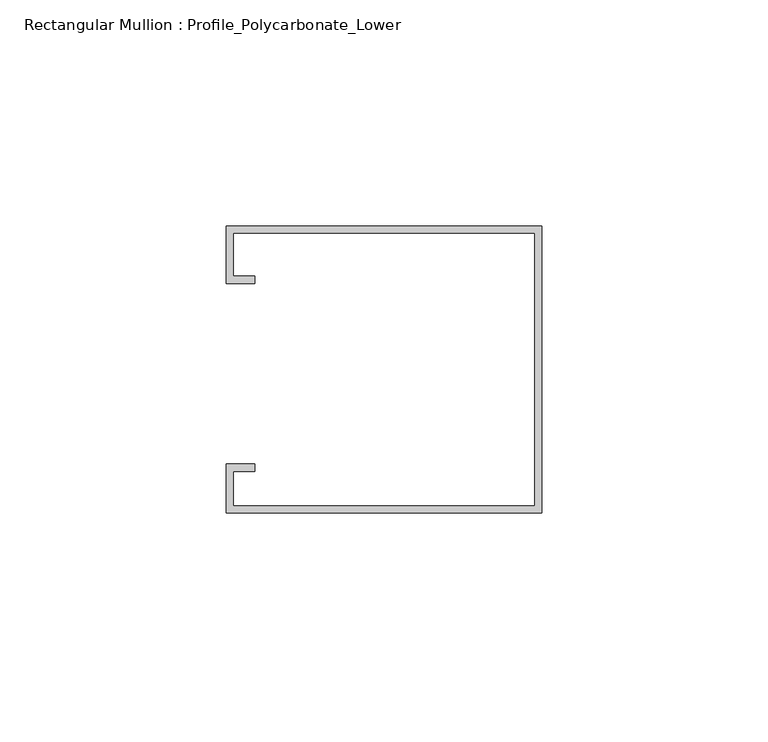
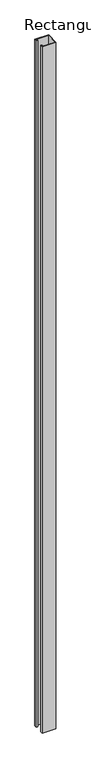
"""IFC4 building model written with IfcOpenShell, lengths in millimetres: member geometry, Rectangular Mullion : Profile_Polycarbonate_Lower."""

from ifc_helpers import new_model, si_unit, frame, origin, place, context, project, spatial, polyline, outline, extrude, source, transform, mapped, element, save


def rectangular_mullion_profile_polycarbonate_lower_9e976f01(model_context):
    return source(origin(), model_context, "Body", "SweptSolid", [
        extrude(outline(polyline([(0.0, 32.7), (0.0, -30.8), (-69.85, -30.8), (-69.85, -20.0), (-63.5, -20.0), (-63.5, -21.5875), (-68.2625, -21.5875), (-68.2625, -29.2125), (-1.5875, -29.2125), (-1.5875, 31.1125), (-68.2625, 31.1125), (-68.2625, 21.5875), (-63.5, 21.5875), (-63.5, 20.0), (-69.85, 20.0), (-69.85, 32.7), (0.0, 32.7)])), frame((0.0, 0.0, -3684.5875), z_axis=(0.0, 0.0, 1.0), x_axis=(1.0, 0.0, 0.0)), (0.0, 0.0, 1.0), 3684.5875),
    ])


if __name__ == "__main__":
    model = new_model("IFC4")
    model_context = context("Model", 3, world=origin())
    ifc_project = project(units=[si_unit("LENGTHUNIT", "METRE", prefix="MILLI")], contexts=[model_context])
    site = spatial("IfcSite", under=ifc_project)
    building = spatial("IfcBuilding", under=site)
    placement = place(None, origin())
    rectangular_mullion_profile_polycarbonate_lower_shape = rectangular_mullion_profile_polycarbonate_lower_9e976f01(model_context)
    element("IfcMember", 1, ObjectType="Rectangular Mullion : Profile_Polycarbonate_Lower", at=placement, inside=building, context=model_context, shape_type="MappedRepresentation", body=[
        mapped(rectangular_mullion_profile_polycarbonate_lower_shape, transform((0.0, 0.0, 0.0), x_axis=(1.0, 0.0, 0.0), y_axis=(0.0, 1.0, 0.0), z_axis=(0.0, 0.0, 1.0))),
    ])
    save(model, "model.ifc")

# Revit data of these elements
# Type "Rectangular Mullion : Profile_Polycarbonate_Lower"
#   built-in parameter 1007322 = 0.208333 (stored number, unit not read)
#   built-in parameter 1007321 = 0 (stored number, unit not read)
#   built-in parameter 1007320 = 0.00520833 (stored number, unit not read)
# Element 1 (IfcMember, "Rectangular Mullion : Profile_Polycarbonate_Lower")
#   Materials on its faces: "ALUMINUM PROFILE AT POLYCARBONATE PANEL"
# Materials
#   "ALUMINUM PROFILE AT POLYCARBONATE PANEL": class "Metal", colour RGB 244 244 244, transparency 0, Description = "Aluminum 6061", Cost = 0
